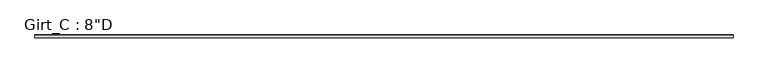
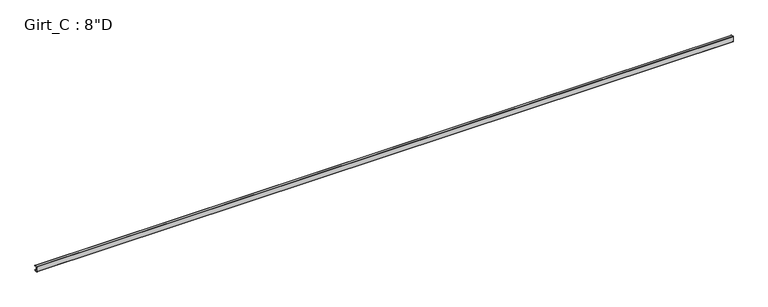
"""IFC4 building model written with IfcOpenShell, lengths in millimetres: beam geometry."""

from ifc_helpers import new_model, si_unit, point, frame, frame_2d, origin, place, context, project, spatial, polyline, circle_curve, trimmed, segment, composite_curve, outline, extrude, source, transform, mapped, element, save


def beam_25f88f39(model_context):
    return source(origin(), model_context, "Body", "SweptSolid", [
        extrude(outline(composite_curve([segment(polyline([(87.5109375, 101.6), (99.7560415, 87.0068534), (97.6278742, 85.221109), (86.2154765, 98.821875), (3.3005807, 98.821875)]), True, "CONTINUOUS"), segment(trimmed(circle_curve(frame_2d((3.3741066, 96.8381931)), 1.9850441), [point((3.3005807, 98.821875))], [point((1.3890625, 96.8381931))], True, "CARTESIAN"), True, "CONTINUOUS"), segment(polyline([(1.3890625, 96.8381931), (1.3890625, -96.8389339)]), True, "CONTINUOUS"), segment(trimmed(circle_curve(frame_2d((3.3748024, -96.8389339)), 1.9857399), [point((1.3890625, -96.8389339))], [point((3.2694106, -98.821875))], True, "CARTESIAN"), True, "CONTINUOUS"), segment(polyline([(3.2694106, -98.821875), (86.2154765, -98.821875), (97.6510975, -85.1934327), (99.7792647, -86.979177), (87.5109375, -101.6), (3.3734375, -101.6)]), True, "CONTINUOUS"), segment(trimmed(circle_curve(frame_2d((3.3734375, -96.8375)), 4.7625), [point((3.3734375, -101.6))], [point((-1.3890625, -96.8375))], False, "CARTESIAN"), True, "CONTINUOUS"), segment(polyline([(-1.3890625, -96.8375), (-1.3890625, 96.8375)]), True, "CONTINUOUS"), segment(trimmed(circle_curve(frame_2d((3.3734375, 96.8375)), 4.7625), [point((-1.3890625, 96.8375))], [point((3.3734375, 101.6))], False, "CARTESIAN"), True, "CONTINUOUS"), segment(polyline([(3.3734375, 101.6), (87.5109375, 101.6)]), True, "CONTINUOUS")], self_intersect=False)), frame((-12866.6875, 0.0, 0.0), z_axis=(1.0, 0.0, 0.0), x_axis=(0.0, 1.0, 0.0)), (0.0, 0.0, 1.0), 25517.475),
    ])


if __name__ == "__main__":
    model = new_model("IFC4")
    model_context = context("Model", 3, world=origin())
    ifc_project = project(units=[si_unit("LENGTHUNIT", "METRE", prefix="MILLI")], contexts=[model_context])
    site = spatial("IfcSite", under=ifc_project)
    building = spatial("IfcBuilding", under=site)
    placement = place(None, origin())
    beam_shape = beam_25f88f39(model_context)
    element("IfcBeam", 1, ObjectType="Girt_C : 8\"D", at=placement, inside=building, context=model_context, shape_type="MappedRepresentation", body=[
        mapped(beam_shape, transform((0.0, 0.0, 0.0), x_axis=(1.0, 0.0, 0.0), y_axis=(0.0, 1.0, 0.0), z_axis=(0.0, 0.0, 1.0))),
    ])
    save(model, "model.ifc")

# Revit data of these elements
# Type "Girt_C : 8\"D"
#   half leg = 0' - 1 3/4"
#   Web_Thickness = 0' - 0 7/64"
#   Length [instance default] = 10' - 0"
#   Leg_1 = 0' - 3 1/2"
#   Height = 0' - 8"
#   Structural Material [instance default] = none
# Element 1 (IfcBeam, "Girt_C : 8\"D")
#   Structural Material = CEE' SECTION (8.0x3.5C - SEE STRUCT. DWGS)
#   Materials on its faces: "CEE' SECTION (8.0x3.5C - SEE STRUCT. DWGS)"
# Materials
#   "CEE' SECTION (8.0x3.5C - SEE STRUCT. DWGS)": class "Metal", colour RGB 137 146 153, transparency 0, Description = "Steel, mill finish", Cost = 0
